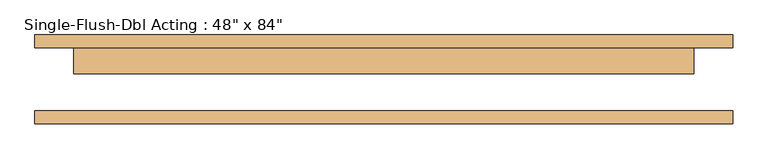
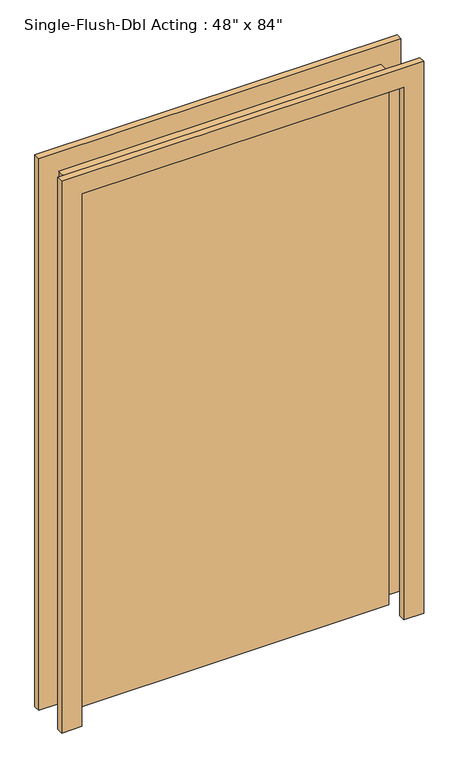
"""IFC4 building model written with IfcOpenShell, lengths in millimetres: door geometry."""

from ifc_helpers import new_model, si_unit, frame, origin, origin_with_axes, place, context, project, spatial, polyline, outline, extrude, source, transform, mapped, element, save


def door_0c2cb489(model_context):
    return source(origin(), model_context, "Body", "SweptSolid", [
        extrude(outline(polyline([(2209.8, -685.8), (0.0, -685.8), (0.0, -609.6), (2133.6, -609.6), (2133.6, 609.6), (0.0, 609.6), (0.0, 685.8), (2209.8, 685.8), (2209.8, -685.8)])), frame((0.0, 61.9125, 0.0), z_axis=(0.0, 1.0, 0.0), x_axis=(0.0, 0.0, 1.0)), (0.0, 0.0, 1.0), 25.4),
        extrude(outline(polyline([(2209.8, 685.8), (2209.8, -685.8), (0.0, -685.8), (0.0, -609.6), (2133.6, -609.6), (2133.6, 609.6), (0.0, 609.6), (0.0, 685.8), (2209.8, 685.8)])), frame((0.0, -87.3125, 0.0), z_axis=(0.0, 1.0, 0.0), x_axis=(0.0, 0.0, 1.0)), (0.0, 0.0, 1.0), 25.4),
        extrude(outline(polyline([(609.6, 11.1125), (-609.6, 11.1125), (-609.6, 61.9125), (609.6, 61.9125), (609.6, 11.1125)])), origin_with_axes(), (0.0, 0.0, 1.0), 2133.6),
    ])


if __name__ == "__main__":
    model = new_model("IFC4")
    model_context = context("Model", 3, world=origin())
    ifc_project = project(units=[si_unit("LENGTHUNIT", "METRE", prefix="MILLI")], contexts=[model_context])
    site = spatial("IfcSite", under=ifc_project)
    building = spatial("IfcBuilding", under=site)
    placement = place(None, origin())
    door_shape = door_0c2cb489(model_context)
    element("IfcDoor", 1, ObjectType="Single-Flush-Dbl Acting : 48\" x 84\"", at=placement, inside=building, context=model_context, shape_type="MappedRepresentation", body=[
        mapped(door_shape, transform((0.0, 0.0, 0.0), x_axis=(1.0, 0.0, 0.0), y_axis=(0.0, 1.0, 0.0), z_axis=(0.0, 0.0, 1.0))),
    ])
    save(model, "model.ifc")

# Revit data of these elements
# Project information
#   Room Abbreviation = "ORGS1"
#   Room Description = "Operating Room, Integrated (ORGS1)"
#   Sheets - Total = "7"
#   Project Issue Date = "Issue Date"
#   Project Status = "Project Status"
#   Client Name = "Owner"
#   Project Address = "Enter address here"
#   Project Name = "Project Name"
#   Project Number = "Project Number"
#   Publication Date = "30-Jan-15"
# Type "Single-Flush-Dbl Acting : 48\" x 84\""
#   Type Mark = "23"
#   Construction Type = "H"
#   Assembly Code = "C1020"
#   Thickness = 0' - 2"
#   Height = 7' - 0"
#   Rail Width - Center = 0' - 4"
#   Trim Projection Ext. = 0' - 1"
#   Trim Projection Int. = 0' - 1"
#   Trim Width Ext. = 0' - 3"
#   Trim Width Int. = 0' - 3"
#   Width = 4' - 0"
#   Door Material = Door - Panel
#   Frame Material = Door - Frame
#   Function = (empty or 0)
#   Wall Closure = (empty or 0)
# Element 1 (IfcDoor, "Single-Flush-Dbl Acting : 48\" x 84\"")
#   Materials on its faces: "Door - Frame", "Door - Panel"
# Materials
#   "Door - Panel": class "Wood", colour RGB 210 159 95, transparency 0
#   "Door - Frame": class "Miscellaneous", colour RGB 118 70 51, transparency 0
